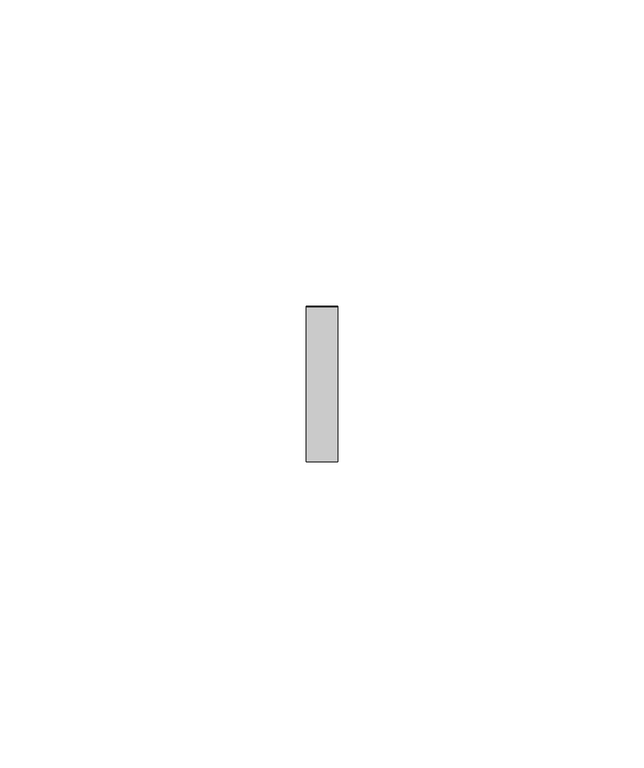
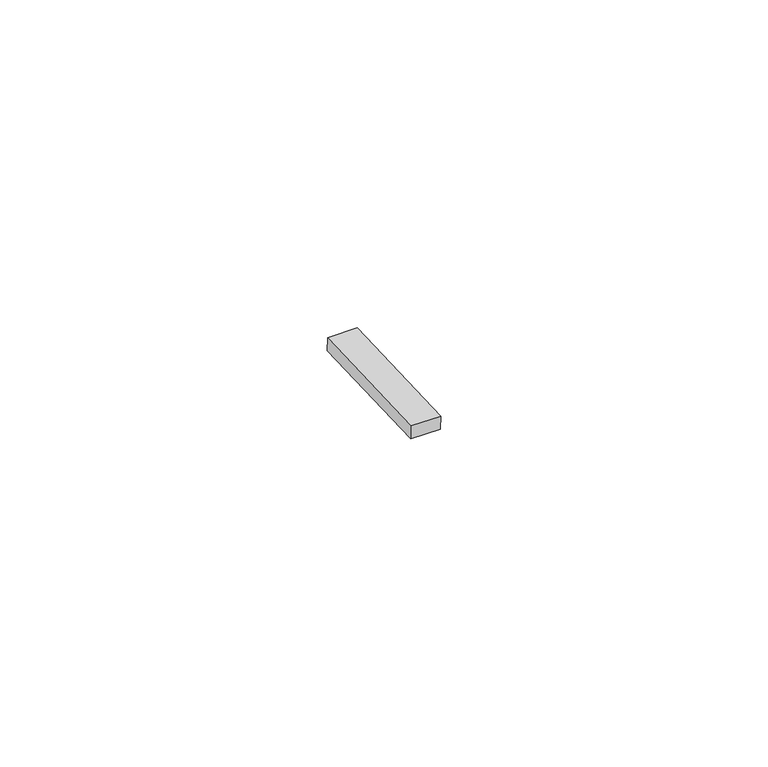
"""IFC4 building model written with IfcOpenShell, lengths in millimetres: proxy geometry, Inner panel:Inner panel:1:Inner panel:1 : Inner panel:Inner panel:300324:2:Inner panel:1:Inner panel:1 : Inner panel:Inner panel:300324:2 : Inner panel:Inner panel:1:Inner panel:1 : Inner panel:Inner panel:300324:300043:56 : Inner panel:Inner panel:1:Inner panel:1 : Inner panel:Inner panel:300324:2:Inner panel:1:Inner panel:1 : Inner panel:Inner panel:300324:2 : Inner panel:Inner panel:1:Inner panel:1 : Inner panel:Inner panel:300324:300043:308120."""

from ifc_helpers import new_model, si_unit, frame, origin, place, context, project, spatial, polyline, outline, extrude, source, transform, mapped, element, save


def generic_models_8c909bb7(model_context):
    return source(origin(), model_context, "Body", "SweptSolid", [
        extrude(outline(polyline([(0.0, -25.3999999), (0.0, 0.0), (5.2138089, 0.0), (5.2138089, -25.3999999), (0.0, -25.3999999)])), frame((593530.195117, -566905.6162814, 8857.0720004), z_axis=(0.0, -0.041630544712223896, 0.9991330730923502), x_axis=(-1.0, 0.0, 0.0)), (0.0, 0.0, 1.0), 2.4763745),
    ])


if __name__ == "__main__":
    model = new_model("IFC4")
    model_context = context("Model", 3, world=origin())
    ifc_project = project(units=[si_unit("LENGTHUNIT", "METRE", prefix="MILLI")], contexts=[model_context])
    site = spatial("IfcSite", under=ifc_project)
    building = spatial("IfcBuilding", under=site)
    placement = place(None, origin())
    generic_models_shape = generic_models_8c909bb7(model_context)
    element("IfcBuildingElementProxy", 1, Name="Inner panel:Inner panel:1:Inner panel:1 : Inner panel:Inner panel:300324:2:Inner panel:1:Inner panel:1 : Inner panel:Inner panel:300324:2 : Inner panel:Inner panel:1:Inner panel:1 : Inner panel:Inner panel:300324:300043:56 : Inner panel:Inner panel:1:Inner panel:1 : Inner panel:Inner panel:300324:2:Inner panel:1:Inner panel:1 : Inner panel:Inner panel:300324:2 : Inner panel:Inner panel:1:Inner panel:1 : Inner panel:Inner panel:300324:300043:308120", ObjectType="Inner panel:Inner panel:1:Inner panel:1 : Inner panel:Inner panel:300324:2:Inner panel:1:Inner panel:1 : Inner panel:Inner panel:300324:2 : Inner panel:Inner panel:1:Inner panel:1 : Inner panel:Inner panel:300324:300043:56 : Inner panel:Inner panel:1:Inner panel:1 : Inner panel:Inner panel:300324:2:Inner panel:1:Inner panel:1 : Inner panel:Inner panel:300324:2 : Inner panel:Inner panel:1:Inner panel:1 : Inner panel:Inner panel:300324:300043:308120", at=placement, inside=building, context=model_context, shape_type="MappedRepresentation", body=[
        mapped(generic_models_shape, transform((0.0, 0.0, 0.0), x_axis=(1.0, 0.0, 0.0), y_axis=(0.0, 1.0, 0.0), z_axis=(0.0, 0.0, 1.0))),
    ])
    save(model, "model.ifc")

# Revit data of these elements
# Type "Inner panel:Inner panel:1:Inner panel:1 : Inner panel:Inner panel:300324:2:Inner panel:1:Inner panel:1 : Inner panel:Inner panel:300324:2 : Inner panel:Inner panel:1:Inner panel:1 : Inner panel:Inner panel:300324:300043:56 : Inner panel:Inner panel:1:Inner panel:1 : Inner panel:Inner panel:300324:2:Inner panel:1:Inner panel:1 : Inner panel:Inner panel:300324:2 : Inner panel:Inner panel:1:Inner panel:1 : Inner panel:Inner panel:300324:300043:308120"
#   NameOverride = "Inner panel:Inner panel:1:Inner panel:1 : Inner panel:Inner panel:300324:2:Inner panel:1:Inner panel:1 : Inner panel:Inner panel:300324:2 : Inner panel:Inner panel:1:Inner panel:1 : Inner panel:Inner panel:300324:300043:308120"
#   ObjectTypeOverride = "Inner panel:1:Inner panel:1 : Inner panel:Inner panel:300324:2 : Inner panel:Inner panel:1:Inner panel:1 : Inner panel:Inner panel:300324:300043"
#   Reference = "Inner panel"
#   Tag = "308120"
# Element 1 (IfcBuildingElementProxy, "Inner panel:Inner panel:1:Inner panel:1 : Inner panel:Inner panel:300324:2:Inner panel:1:Inner panel:1 : Inner panel:Inner panel:300324:2 : Inner panel:Inner panel:1:Inner panel:1 : Inner panel:Inner panel:300324:300043:56 : Inner panel:Inner panel:1:Inner panel:1 : Inner panel:Inner panel:300324:2:Inner panel:1:Inner panel:1 : Inner panel:Inner panel:300324:2 : Inner panel:Inner panel:1:Inner panel:1 : Inner panel:Inner panel:300324:300043:308120")
#   Materials on its faces: "AT CLIP - 1\" WIDE NON ABSORBENT, WEATHER-RESISTANT NEOPRENE/EPDM/SBR FOAM"
# Materials
#   "AT CLIP - 1\" WIDE NON ABSORBENT, WEATHER-RESISTANT NEOPRENE/EPDM/SBR FOAM": class "Generic", colour RGB 85 85 85, transparency 0, Cost = 0
